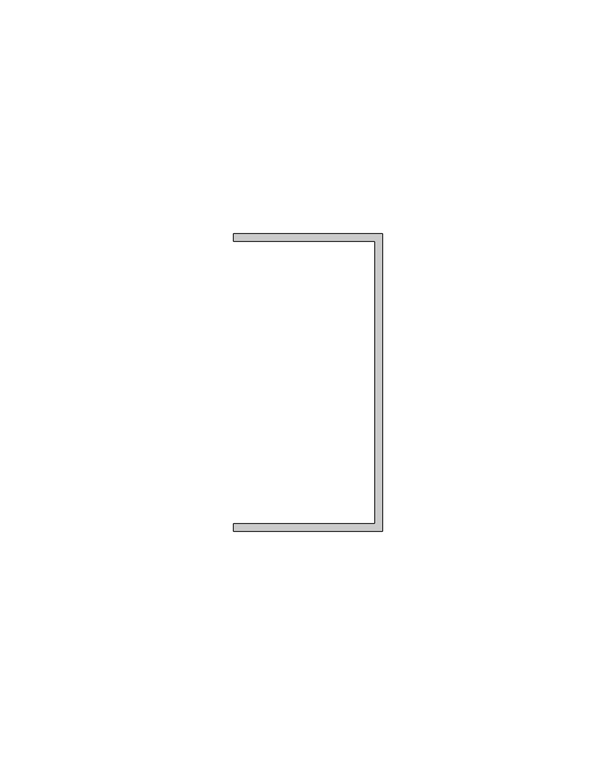
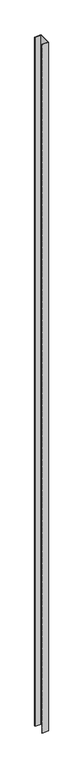
"""IFC4 building model written with IfcOpenShell, lengths in millimetres: proxy geometry, Generic Models 7:Generic Models 1:3:Generic Models 1:3 : Generic Models 7:Generic Models 1:305549:3:Generic Models 1:3:Generic Models 1:3 : Generic Models 7:Generic Models 1:305549:3 : Generic Models 7:Generic Models 1:3:Generic Models 1:3 : Generic Models 7:Generic Models 1:305549:301244:6 : Generic Models 7:Generic Models 1:3:Generic Models 1:3 : Generic Models 7:Generic Models 1:305549:3:Generic Models 1:3:Generic Models 1:3 : Generic Models 7:Generic Models 1:305549:3 : Generic Models 7:Generic Models 1:3:Generic Models 1:3 : Generic Models 7:Generic Models 1:305549:301244:308848."""

from ifc_helpers import new_model, si_unit, frame, origin, place, context, project, spatial, polyline, outline, extrude, source, transform, mapped, element, save


def generic_models_b91b884d(model_context):
    return source(origin(), model_context, "Body", "SweptSolid", [
        extrude(outline(polyline([(570446.4412361, -579013.3913841), (570446.4412361, -579076.8913841), (570414.6912361, -579076.8913841), (570414.6912361, -579075.3038841), (570444.8537361, -579075.3038841), (570444.8537361, -579014.9788841), (570414.6912361, -579014.9788841), (570414.6912361, -579013.3913841), (570446.4412361, -579013.3913841)])), frame((0.0, 0.0, 38.1), z_axis=(0.0, 0.0, 1.0), x_axis=(1.0, 0.0, 0.0)), (0.0, 0.0, 1.0), 3657.6),
    ])


if __name__ == "__main__":
    model = new_model("IFC4")
    model_context = context("Model", 3, world=origin())
    ifc_project = project(units=[si_unit("LENGTHUNIT", "METRE", prefix="MILLI")], contexts=[model_context])
    site = spatial("IfcSite", under=ifc_project)
    building = spatial("IfcBuilding", under=site)
    placement = place(None, origin())
    generic_models_shape = generic_models_b91b884d(model_context)
    element("IfcBuildingElementProxy", 1, Name="Generic Models 7:Generic Models 1:3:Generic Models 1:3 : Generic Models 7:Generic Models 1:305549:3:Generic Models 1:3:Generic Models 1:3 : Generic Models 7:Generic Models 1:305549:3 : Generic Models 7:Generic Models 1:3:Generic Models 1:3 : Generic Models 7:Generic Models 1:305549:301244:6 : Generic Models 7:Generic Models 1:3:Generic Models 1:3 : Generic Models 7:Generic Models 1:305549:3:Generic Models 1:3:Generic Models 1:3 : Generic Models 7:Generic Models 1:305549:3 : Generic Models 7:Generic Models 1:3:Generic Models 1:3 : Generic Models 7:Generic Models 1:305549:301244:308848", ObjectType="Generic Models 7:Generic Models 1:3:Generic Models 1:3 : Generic Models 7:Generic Models 1:305549:3:Generic Models 1:3:Generic Models 1:3 : Generic Models 7:Generic Models 1:305549:3 : Generic Models 7:Generic Models 1:3:Generic Models 1:3 : Generic Models 7:Generic Models 1:305549:301244:6 : Generic Models 7:Generic Models 1:3:Generic Models 1:3 : Generic Models 7:Generic Models 1:305549:3:Generic Models 1:3:Generic Models 1:3 : Generic Models 7:Generic Models 1:305549:3 : Generic Models 7:Generic Models 1:3:Generic Models 1:3 : Generic Models 7:Generic Models 1:305549:301244:308848", at=placement, inside=building, context=model_context, shape_type="MappedRepresentation", body=[
        mapped(generic_models_shape, transform((0.0, 0.0, 0.0), x_axis=(1.0, 0.0, 0.0), y_axis=(0.0, 1.0, 0.0), z_axis=(0.0, 0.0, 1.0))),
    ])
    save(model, "model.ifc")

# Revit data of these elements
# Type "Generic Models 7:Generic Models 1:3:Generic Models 1:3 : Generic Models 7:Generic Models 1:305549:3:Generic Models 1:3:Generic Models 1:3 : Generic Models 7:Generic Models 1:305549:3 : Generic Models 7:Generic Models 1:3:Generic Models 1:3 : Generic Models 7:Generic Models 1:305549:301244:6 : Generic Models 7:Generic Models 1:3:Generic Models 1:3 : Generic Models 7:Generic Models 1:305549:3:Generic Models 1:3:Generic Models 1:3 : Generic Models 7:Generic Models 1:305549:3 : Generic Models 7:Generic Models 1:3:Generic Models 1:3 : Generic Models 7:Generic Models 1:305549:301244:308848"
#   NameOverride = "Generic Models 7:Generic Models 1:3:Generic Models 1:3 : Generic Models 7:Generic Models 1:305549:3:Generic Models 1:3:Generic Models 1:3 : Generic Models 7:Generic Models 1:305549:3 : Generic Models 7:Generic Models 1:3:Generic Models 1:3 : Generic Models 7:Generic Models 1:305549:301244:308848"
#   ObjectTypeOverride = "Generic Models 1:3:Generic Models 1:3 : Generic Models 7:Generic Models 1:305549:3 : Generic Models 7:Generic Models 1:3:Generic Models 1:3 : Generic Models 7:Generic Models 1:305549:301244"
#   Reference = "Generic Models 1"
#   Tag = "308848"
# Element 1 (IfcBuildingElementProxy, "Generic Models 7:Generic Models 1:3:Generic Models 1:3 : Generic Models 7:Generic Models 1:305549:3:Generic Models 1:3:Generic Models 1:3 : Generic Models 7:Generic Models 1:305549:3 : Generic Models 7:Generic Models 1:3:Generic Models 1:3 : Generic Models 7:Generic Models 1:305549:301244:6 : Generic Models 7:Generic Models 1:3:Generic Models 1:3 : Generic Models 7:Generic Models 1:305549:3:Generic Models 1:3:Generic Models 1:3 : Generic Models 7:Generic Models 1:305549:3 : Generic Models 7:Generic Models 1:3:Generic Models 1:3 : Generic Models 7:Generic Models 1:305549:301244:308848")
#   Materials on its faces: "GALVANIZED U-CHANNEL (250T125-33)"
# Materials
#   "GALVANIZED U-CHANNEL (250T125-33)": class "Unassigned", colour RGB 202 201 200, transparency 0, Keynote = "M05451300.02", Cost = 0
